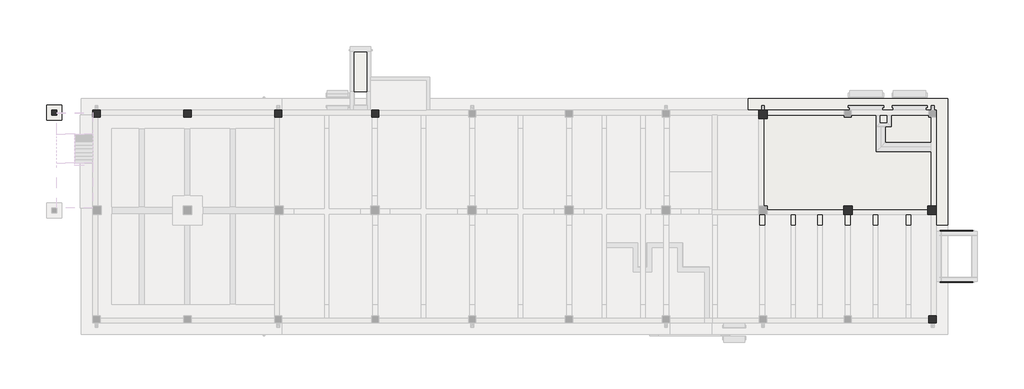
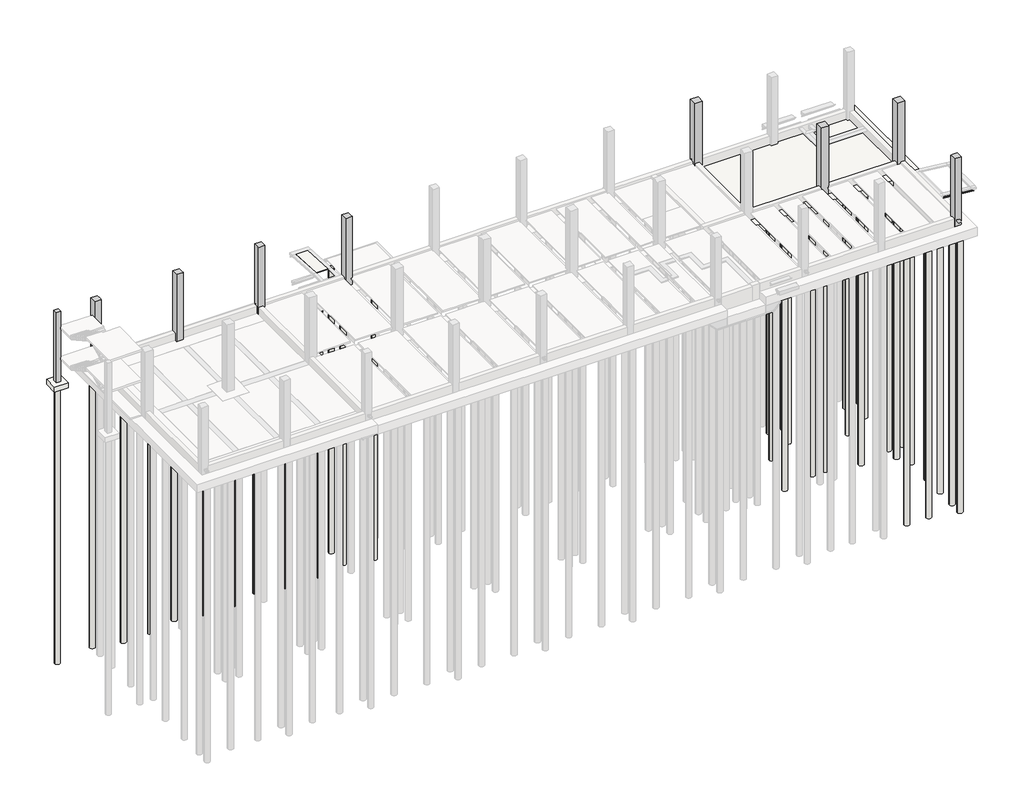
# One storey, part 6 of 7: 46 slabs, 9 columns.
"""IFC4 building model written with IfcOpenShell, lengths in millimetres."""

from ifc_helpers import new_model, si_unit, point, frame, frame_2d, origin, place, context, project, spatial, polyline, circle_curve, trimmed, segment, composite_curve, outline, extrude, faceted_brep, element, save

model = new_model("IFC4")

# Units and contexts
model_context = context("Model", 3, world=origin())
ifc_project = project(units=[si_unit("LENGTHUNIT", "METRE", prefix="MILLI")], contexts=[model_context])

# Site, building, storey
site = spatial("IfcSite", under=ifc_project)
building = spatial("IfcBuilding", under=site)
storey = spatial("IfcBuildingStorey", under=building, Name="H.P.P", Elevation=4500.0)

# Columns
placement = place(None, origin())
element("IfcColumn", 1, ObjectType="RC_Column_Rectangular : H_SC_AR S15_RC Col-AG_700x700_C1", at=placement, inside=storey, context=model_context, shape_type="Brep", body=[
    faceted_brep([(62350.0, -7650.0, 4000.0), (62350.0, -7950.0, 4000.0), (62350.0, -8350.0, 4000.0), (61650.0, -8350.0, 4000.0), (61650.0, -7950.0, 4000.0), (61650.0, -7650.0, 4000.0), (62350.0, -7650.0, 10600.0), (62350.0, -8350.0, 10600.0), (62350.0, -8350.0, 10450.0), (62350.0, -8350.0, 4800.0), (62350.0, -8350.0, 4650.0), (62250.0, -8350.0, 10600.0), (61750.0, -8350.0, 10600.0), (61650.0, -8350.0, 10600.0), (61650.0, -8350.0, 10450.0), (61650.0, -8350.0, 4800.0), (61650.0, -8350.0, 4650.0), (61650.0, -7650.0, 10600.0)], [[[0, 1, 2, 3, 4, 5]], [[2, 1, 0, 6, 7, 8, 9, 10]], [[3, 2, 10, 9, 8, 7, 11, 12, 13, 14, 15, 16]], [[5, 4, 3, 16, 15, 14, 13, 17]], [[0, 5, 17, 6]], [[7, 6, 17, 13, 12, 11]]]),
])
element("IfcColumn", 2, ObjectType="RC_Column_Rectangular : H_SC_AR S15_RC Col-AG_700x700_C1", at=placement, inside=storey, context=model_context, shape_type="Brep", body=[
    faceted_brep([(69300.0, -7650.0, 4000.0), (69300.0, -8350.0, 4000.0), (68900.0, -8350.0, 4000.0), (68600.0, -8350.0, 4000.0), (68600.0, -7950.0, 4000.0), (68600.0, -7650.0, 4000.0), (68900.0, -7650.0, 4000.0), (69300.0, -7650.0, 4800.0), (69300.0, -7650.0, 9900.0), (69300.0, -7650.0, 10600.0), (69300.0, -8350.0, 10600.0), (69300.0, -8350.0, 9900.0), (69300.0, -8350.0, 4800.0), (68900.0, -8350.0, 10600.0), (68600.0, -8350.0, 10600.0), (68600.0, -8350.0, 10450.0), (68600.0, -8350.0, 9800.0), (68600.0, -8350.0, 4800.0), (68600.0, -8350.0, 4650.0), (68600.0, -7650.0, 10600.0)], [[[0, 1, 2, 3, 4, 5, 6]], [[1, 0, 7, 8, 9, 10, 11, 12]], [[3, 2, 1, 12, 11, 10, 13, 14, 15, 16, 17, 18]], [[5, 4, 3, 18, 17, 16, 15, 14, 19]], [[0, 6, 5, 19, 9, 8, 7]], [[10, 9, 19, 14, 13]]]),
])
element("IfcColumn", 3, ObjectType="RC_Column_Rectangular : H_SC_AR S15_RC Col-AG_700x700_C1", at=placement, inside=storey, context=model_context, shape_type="Brep", body=[
    faceted_brep([(55350.0, 300.0, 4000.0), (55350.0, -100.0, 4000.0), (55350.0, -400.0, 4000.0), (55050.0, -400.0, 4000.0), (54650.0, -400.0, 4000.0), (54650.0, -100.0, 4000.0), (54650.0, 300.0, 4000.0), (55350.0, 300.0, 10600.0), (55350.0, -400.0, 10600.0), (55350.0, 300.0, 4800.0), (55350.0, 300.0, 8300.0), (55350.0, 300.0, 9100.0), (54650.0, -400.0, 10600.0), (54650.0, -400.0, 9800.0), (54650.0, -400.0, 4800.0), (54650.0, 300.0, 10600.0), (54650.0, 300.0, 9800.0), (54650.0, 300.0, 4800.0)], [[[0, 1, 2, 3, 4, 5, 6]], [[7, 8, 2, 1, 0, 9, 10, 11]], [[8, 12, 13, 14, 4, 3, 2]], [[12, 15, 16, 17, 6, 5, 4, 14, 13]], [[15, 7, 11, 10, 9, 0, 6, 17, 16]], [[7, 15, 12, 8]]]),
])
element("IfcColumn", 4, ObjectType="RC_Column_Rectangular : H_SC_AR S15_RC Col-AG_600x600_C2", at=placement, inside=storey, context=model_context, shape_type="Brep", body=[
    faceted_brep([(300.0, 300.0, 4100.0), (300.0, -100.0, 4100.0), (300.0, -300.0, 4100.0), (100.0, -300.0, 4100.0), (-300.0, -300.0, 4100.0), (-300.0, -100.0, 4100.0), (-300.0, 300.0, 4100.0), (300.0, 300.0, 4800.0), (300.0, 300.0, 9800.0), (300.0, 300.0, 10600.0), (300.0, -100.0, 10600.0), (300.0, -300.0, 10600.0), (300.0, -300.0, 10450.0), (100.0, -300.0, 10600.0), (-300.0, -300.0, 10600.0), (-300.0, -300.0, 9900.0), (-300.0, -300.0, 4800.0), (-300.0, 300.0, 10600.0), (-300.0, 300.0, 10550.0), (-300.0, 300.0, 9950.0), (-300.0, 300.0, 4630.0)], [[[0, 1, 2, 3, 4, 5, 6]], [[2, 1, 0, 7, 8, 9, 10, 11, 12]], [[4, 3, 2, 12, 11, 13, 14, 15, 16]], [[6, 5, 4, 16, 15, 14, 17, 18, 19, 20]], [[0, 6, 20, 19, 18, 17, 9, 8, 7]], [[17, 14, 13, 11, 10, 9]]]),
])
element("IfcColumn", 5, ObjectType="RC_Column_Rectangular : H_SC_AR S15_RC Col-AG_600x600_C2", at=placement, inside=storey, context=model_context, shape_type="Brep", body=[
    faceted_brep([(7800.0, 300.0, 4100.0), (7800.0, -100.0, 4100.0), (7800.0, -300.0, 4100.0), (7200.0, -300.0, 4100.0), (7200.0, -100.0, 4100.0), (7200.0, 300.0, 4100.0), (7800.0, 300.0, 4800.0), (7800.0, 300.0, 9800.0), (7800.0, 300.0, 10600.0), (7800.0, -100.0, 10600.0), (7800.0, -300.0, 10600.0), (7800.0, -300.0, 10450.0), (7750.0, -300.0, 10600.0), (7250.0, -300.0, 10600.0), (7200.0, -300.0, 10600.0), (7200.0, -300.0, 10450.0), (7200.0, -100.0, 10600.0), (7200.0, 300.0, 10600.0), (7200.0, 300.0, 9800.0), (7200.0, 300.0, 4800.0)], [[[0, 1, 2, 3, 4, 5]], [[2, 1, 0, 6, 7, 8, 9, 10, 11]], [[3, 2, 11, 10, 12, 13, 14, 15]], [[5, 4, 3, 15, 14, 16, 17, 18, 19]], [[0, 5, 19, 18, 17, 8, 7, 6]], [[8, 17, 16, 14, 13, 12, 10, 9]]]),
])
element("IfcColumn", 6, ObjectType="RC_Column_Rectangular : H_SC_AR S15_RC Col-AG_600x600_C2", at=placement, inside=storey, context=model_context, shape_type="Brep", body=[
    faceted_brep([(15300.0, 300.0, 4100.0), (15300.0, -300.0, 4100.0), (15100.0, -300.0, 4100.0), (14700.0, -300.0, 4100.0), (14700.0, -100.0, 4100.0), (14700.0, 300.0, 4100.0), (15300.0, 300.0, 4800.0), (15300.0, 300.0, 9800.0), (15300.0, 300.0, 10600.0), (15300.0, -100.0, 10600.0), (15300.0, -300.0, 10600.0), (15300.0, -300.0, 10450.0), (15300.0, -300.0, 4800.0), (15300.0, -300.0, 4650.0), (15200.0, -300.0, 10600.0), (14700.0, -300.0, 10600.0), (14700.0, -300.0, 10450.0), (14700.0, -300.0, 4800.0), (14700.0, -100.0, 10600.0), (14700.0, 300.0, 10600.0), (14700.0, 300.0, 9800.0), (14700.0, 300.0, 4800.0)], [[[0, 1, 2, 3, 4, 5]], [[1, 0, 6, 7, 8, 9, 10, 11, 12, 13]], [[3, 2, 1, 13, 12, 11, 10, 14, 15, 16, 17]], [[5, 4, 3, 17, 16, 15, 18, 19, 20, 21]], [[0, 5, 21, 20, 19, 8, 7, 6]], [[8, 19, 18, 15, 14, 10, 9]]]),
])
element("IfcColumn", 7, ObjectType="RC_Column_Rectangular : H_SC_AR S15_RC Col-AG_600x600_C2", at=placement, inside=storey, context=model_context, shape_type="Brep", body=[
    faceted_brep([(23300.0, 300.0, 4000.0), (23300.0, -100.0, 4000.0), (23300.0, -300.0, 4000.0), (22700.0, -300.0, 4000.0), (22700.0, -100.0, 4000.0), (22700.0, 300.0, 4000.0), (23300.0, 300.0, 4800.0), (23300.0, 300.0, 9800.0), (23300.0, 300.0, 10600.0), (23300.0, -100.0, 10600.0), (23300.0, -300.0, 10600.0), (23300.0, -300.0, 10450.0), (23300.0, -300.0, 4800.0), (23300.0, -300.0, 4650.0), (23200.0, -300.0, 10600.0), (22700.0, -300.0, 10600.0), (22700.0, -300.0, 10450.0), (22700.0, -300.0, 4800.0), (22700.0, -300.0, 4650.0), (22700.0, -100.0, 10600.0), (22700.0, 300.0, 10600.0), (22700.0, 300.0, 4800.0)], [[[0, 1, 2, 3, 4, 5]], [[2, 1, 0, 6, 7, 8, 9, 10, 11, 12, 13]], [[3, 2, 13, 12, 11, 10, 14, 15, 16, 17, 18]], [[5, 4, 3, 18, 17, 16, 15, 19, 20, 21]], [[0, 5, 21, 20, 8, 7, 6]], [[8, 20, 19, 15, 14, 10, 9]]]),
])
element("IfcColumn", 8, ObjectType="RC_Column_Rectangular : H_SC_AR S15_RC Col-AG_600x600_C2", at=placement, inside=storey, context=model_context, shape_type="Brep", body=[
    faceted_brep([(69300.0, -16700.0, 4000.0), (69300.0, -17300.0, 4000.0), (68700.0, -17300.0, 4000.0), (68700.0, -16900.0, 4000.0), (68700.0, -16700.0, 4000.0), (68900.0, -16700.0, 4000.0), (69300.0, -16700.0, 4800.0), (69300.0, -16700.0, 9900.0), (69300.0, -16700.0, 10600.0), (69300.0, -17300.0, 10600.0), (68700.0, -17300.0, 10600.0), (68700.0, -17300.0, 9800.0), (68700.0, -17300.0, 4800.0), (68700.0, -16900.0, 10600.0), (68700.0, -16700.0, 10600.0), (68700.0, -16700.0, 10450.0), (68700.0, -16700.0, 4800.0), (68700.0, -16700.0, 4650.0), (68900.0, -16700.0, 10600.0)], [[[0, 1, 2, 3, 4, 5]], [[1, 0, 6, 7, 8, 9]], [[2, 1, 9, 10, 11, 12]], [[4, 3, 2, 12, 11, 10, 13, 14, 15, 16, 17]], [[0, 5, 4, 17, 16, 15, 14, 18, 8, 7, 6]], [[9, 8, 18, 14, 13, 10]]]),
])
element("IfcColumn", 9, ObjectType="RC_Column_Rectangular : H_SC_AR S15_RC Col-AG_400x400_C3", at=placement, inside=storey, context=model_context, shape_type="Brep", body=[
    faceted_brep([(-3300.0, 300.0, 3800.0), (-3300.0, -100.0, 3800.0), (-3700.0, -100.0, 3800.0), (-3700.0, 300.0, 3800.0), (-3300.0, 300.0, 10600.0), (-3300.0, -100.0, 10600.0), (-3300.0, -100.0, 10550.0), (-3300.0, -100.0, 9950.0), (-3300.0, -100.0, 7590.0), (-3300.0, -100.0, 6990.0), (-3300.0, -100.0, 4630.0), (-3300.0, -100.0, 4100.0), (-3300.0, -100.0, 4030.0), (-3300.0, 300.0, 4100.0), (-3300.0, 300.0, 4630.0), (-3300.0, 300.0, 9950.0), (-3300.0, 300.0, 10550.0), (-3700.0, -100.0, 10600.0), (-3700.0, -100.0, 10550.0), (-3700.0, -100.0, 9950.0), (-3700.0, -100.0, 7590.0), (-3700.0, -100.0, 6990.0), (-3700.0, -100.0, 4630.0), (-3700.0, -100.0, 4030.0), (-3700.0, 300.0, 10600.0)], [[[0, 1, 2, 3]], [[4, 5, 6, 7, 8, 9, 10, 11, 12, 1, 0, 13, 14, 15, 16]], [[5, 17, 18, 19, 20, 21, 22, 23, 2, 1, 12, 11, 10, 9, 8, 7, 6]], [[17, 24, 3, 2, 23, 22, 21, 20, 19, 18]], [[24, 4, 16, 15, 14, 13, 0, 3]], [[4, 24, 17, 5]]]),
])

# Slabs
element("IfcSlab", 10, ObjectType="H_SF_AR S18_MAT_T800_MF1", at=placement, inside=storey, context=model_context, shape_type="Brep", body=[
    faceted_brep([(70250.0, 1249.9999999, 3200.0), (70250.0, -9250.0000001, 3200.0), (67750.0000002, -9250.0000001, 3200.0), (53749.9998007, -9250.0000001, 3200.0), (53749.9998007, -6750.0000001, 3200.0), (53749.9998007, -1250.0000001, 3200.0), (53749.9998007, 1249.9999999, 3200.0), (70250.0, -9250.0000001, 4000.0), (70250.0, 1249.9999999, 4000.0), (53749.9998007, 1249.9999999, 4000.0), (53749.9998007, -1250.0000001, 4000.0), (53749.9998007, -6750.0000001, 4000.0), (53749.9998007, -9250.0000001, 4000.0), (67750.0000002, -9250.0000001, 4000.0)], [[[0, 1, 2, 3, 4, 5, 6]], [[7, 8, 9, 10, 11, 12, 13]], [[1, 0, 8, 7]], [[1, 7, 13, 12, 3, 2]], [[3, 12, 11, 10, 9, 6, 5, 4]], [[0, 6, 9, 8]]]),
])
element("IfcSlab", 11, ObjectType="H_SF_AR_S18_Lean_T50", at=placement, inside=storey, context=model_context, shape_type="Brep", body=[
    faceted_brep([(72401.1499651, -13950.0, 4178.1393567), (69580.8773013, -13950.0, 4460.1666231), (69580.8773013, -13700.0, 4460.1666231), (72401.1499651, -13700.0, 4178.1393567), (69626.5585541, -13700.0, 4505.847876), (69626.5585541, -13850.0, 4505.847876), (69626.5585541, -13950.0, 4505.847876), (72345.3173228, -13950.0, 4233.9719991), (72345.3173228, -13850.0, 4233.9719991), (72345.3173228, -13700.0, 4233.9719991)], [[[0, 1, 2, 3]], [[4, 5, 6, 7, 8, 9]], [[1, 0, 7, 6]], [[3, 2, 4, 9]], [[5, 4, 2, 1, 6]], [[0, 3, 9, 8, 7]]]),
])
element("IfcSlab", 12, ObjectType="H_SF_AR_S18_Lean_T50", at=placement, inside=storey, context=model_context, shape_type="Brep", body=[
    faceted_brep([(69580.8773013, -9650.0, 4460.1666231), (72401.1499651, -9650.0, 4178.1393567), (72401.1499651, -9900.0, 4178.1393567), (69580.8773013, -9900.0, 4460.1666231), (72345.3173228, -9750.0, 4233.9719991), (72345.3173228, -9650.0, 4233.9719991), (69626.5585541, -9650.0, 4505.847876), (69626.5585541, -9750.0, 4505.847876), (69626.5585541, -9900.0, 4505.847876), (72345.3173228, -9900.0, 4233.9719991)], [[[0, 1, 2, 3]], [[4, 5, 6, 7, 8, 9]], [[1, 0, 6, 5]], [[3, 2, 9, 8]], [[2, 1, 5, 4, 9]], [[0, 3, 8, 7, 6]]]),
])
element("IfcSlab", 13, ObjectType="H_SF_AR_S18_Lean_T50", at=placement, inside=storey, context=model_context, shape_type="Brep", body=[
    faceted_brep([(22338.0, 5100.0, 4329.5560483), (22338.0, 1800.0, 4549.5560483), (21238.0, 1800.0, 4549.5560483), (21238.0, 5100.0, 4329.5560483), (22338.0, 5100.0, 4379.6670362), (21238.0, 5100.0, 4379.6670362), (21238.0, 1800.0, 4599.6670362), (22338.0, 1800.0, 4599.6670362), (22338.0, 1800.0, 4550.0), (21238.0, 1800.0, 4550.0)], [[[0, 1, 2, 3]], [[4, 5, 6, 7]], [[1, 0, 4, 7, 8]], [[2, 1, 8, 7, 6, 9]], [[3, 2, 9, 6, 5]], [[0, 3, 5, 4]]]),
])
element("IfcSlab", 14, ObjectType="Foundation Rectangular (Non-Pile) : H_SF_AR S18_Ret Fdn_1250x1250xT500_F2", at=placement, inside=storey, context=model_context, shape_type="SweptSolid", body=[
    extrude(outline(polyline([(-2875.0, 725.0), (-2875.0, -525.0), (-4125.0, -525.0), (-4125.0, 725.0), (-2875.0, 725.0)])), frame((0.0, 0.0, 3300.0), z_axis=(0.0, 0.0, 1.0), x_axis=(1.0, 0.0, 0.0)), (0.0, 0.0, 1.0), 500.0),
])
element("IfcSlab", 15, ObjectType="PILE : H_FL_AR S19_Pile_D500_L26.9", at=placement, inside=storey, context=model_context, shape_type="SweptSolid", body=[
    extrude(outline(composite_curve([segment(trimmed(circle_curve(frame_2d((-3500.0, 100.0)), 250.0), [point((-3250.0, 100.0))], [point((-3750.0, 100.0))], False, "CARTESIAN"), True, "CONTINUOUS"), segment(trimmed(circle_curve(frame_2d((-3500.0, 100.0)), 250.0), [point((-3750.0, 100.0))], [point((-3250.0, 100.0))], False, "CARTESIAN"), True, "CONTINUOUS")], self_intersect=False)), frame((0.0, 0.0, 3300.0), z_axis=(0.0, 0.0, 1.0), x_axis=(1.0, 0.0, 0.0)), (0.0, 0.0, 1.0), 100.0),
    extrude(outline(composite_curve([segment(trimmed(circle_curve(frame_2d((-3500.0, 100.0)), 250.0), [point((-3750.0, 100.0))], [point((-3250.0, 100.0))], False, "CARTESIAN"), True, "CONTINUOUS"), segment(trimmed(circle_curve(frame_2d((-3500.0, 100.0)), 250.0), [point((-3250.0, 100.0))], [point((-3750.0, 100.0))], False, "CARTESIAN"), True, "CONTINUOUS")], self_intersect=False)), frame((0.0, 0.0, -23500.0), z_axis=(0.0, 0.0, 1.0), x_axis=(1.0, 0.0, 0.0)), (0.0, 0.0, 1.0), 26750.0),
])
element("IfcSlab", 16, ObjectType="PILE : H_FL_AR S19_Pile_D500_L26.9", at=placement, inside=storey, context=model_context, shape_type="SweptSolid", body=[
    extrude(outline(composite_curve([segment(trimmed(circle_curve(frame_2d((0.0, 624.9999997)), 250.0), [point((-250.0, 624.9999997))], [point((250.0, 624.9999997))], False, "CARTESIAN"), True, "CONTINUOUS"), segment(trimmed(circle_curve(frame_2d((0.0, 624.9999997)), 250.0), [point((250.0, 624.9999997))], [point((-250.0, 624.9999997))], False, "CARTESIAN"), True, "CONTINUOUS")], self_intersect=False)), frame((0.0, 0.0, -23500.0), z_axis=(0.0, 0.0, 1.0), x_axis=(1.0, 0.0, 0.0)), (0.0, 0.0, 1.0), 26750.0),
])
element("IfcSlab", 17, ObjectType="PILE : H_FL_AR S19_Pile_D500_L26.9", at=placement, inside=storey, context=model_context, shape_type="SweptSolid", body=[
    extrude(outline(composite_curve([segment(trimmed(circle_curve(frame_2d((2500.0000001, 0.0)), 250.0), [point((2250.0000001, 0.0))], [point((2750.0000001, 0.0))], False, "CARTESIAN"), True, "CONTINUOUS"), segment(trimmed(circle_curve(frame_2d((2500.0000001, 0.0)), 250.0), [point((2750.0000001, 0.0))], [point((2250.0000001, 0.0))], False, "CARTESIAN"), True, "CONTINUOUS")], self_intersect=False)), frame((0.0, 0.0, -23500.0), z_axis=(0.0, 0.0, 1.0), x_axis=(1.0, 0.0, 0.0)), (0.0, 0.0, 1.0), 26750.0),
])
element("IfcSlab", 18, ObjectType="PILE : H_FL_AR S19_Pile_D500_L26.9", at=placement, inside=storey, context=model_context, shape_type="SweptSolid", body=[
    extrude(outline(composite_curve([segment(trimmed(circle_curve(frame_2d((5000.0000002, 0.0)), 250.0), [point((4750.0000002, 0.0))], [point((5250.0000002, 0.0))], False, "CARTESIAN"), True, "CONTINUOUS"), segment(trimmed(circle_curve(frame_2d((5000.0000002, 0.0)), 250.0), [point((5250.0000002, 0.0))], [point((4750.0000002, 0.0))], False, "CARTESIAN"), True, "CONTINUOUS")], self_intersect=False)), frame((0.0, 0.0, -23500.0), z_axis=(0.0, 0.0, 1.0), x_axis=(1.0, 0.0, 0.0)), (0.0, 0.0, 1.0), 26750.0),
])
element("IfcSlab", 19, ObjectType="PILE : H_FL_AR S19_Pile_D500_L26.9", at=placement, inside=storey, context=model_context, shape_type="SweptSolid", body=[
    extrude(outline(composite_curve([segment(trimmed(circle_curve(frame_2d((7500.0, 625.0)), 250.0), [point((7250.0, 625.0))], [point((7750.0, 625.0))], False, "CARTESIAN"), True, "CONTINUOUS"), segment(trimmed(circle_curve(frame_2d((7500.0, 625.0)), 250.0), [point((7750.0, 625.0))], [point((7250.0, 625.0))], False, "CARTESIAN"), True, "CONTINUOUS")], self_intersect=False)), frame((0.0, 0.0, -23500.0), z_axis=(0.0, 0.0, 1.0), x_axis=(1.0, 0.0, 0.0)), (0.0, 0.0, 1.0), 26750.0),
])
element("IfcSlab", 20, ObjectType="PILE : H_FL_AR S19_Pile_D500_L26.9", at=placement, inside=storey, context=model_context, shape_type="SweptSolid", body=[
    extrude(outline(composite_curve([segment(trimmed(circle_curve(frame_2d((10000.0000005, 0.0)), 250.0), [point((9750.0000005, 0.0))], [point((10250.0000005, 0.0))], False, "CARTESIAN"), True, "CONTINUOUS"), segment(trimmed(circle_curve(frame_2d((10000.0000005, 0.0)), 250.0), [point((10250.0000005, 0.0))], [point((9750.0000005, 0.0))], False, "CARTESIAN"), True, "CONTINUOUS")], self_intersect=False)), frame((0.0, 0.0, -23500.0), z_axis=(0.0, 0.0, 1.0), x_axis=(1.0, 0.0, 0.0)), (0.0, 0.0, 1.0), 26750.0),
])
element("IfcSlab", 21, ObjectType="PILE : H_FL_AR S19_Pile_D500_L26.9", at=placement, inside=storey, context=model_context, shape_type="SweptSolid", body=[
    extrude(outline(composite_curve([segment(trimmed(circle_curve(frame_2d((12500.0000007, 0.0)), 250.0), [point((12250.0000007, 0.0))], [point((12750.0000007, 0.0))], False, "CARTESIAN"), True, "CONTINUOUS"), segment(trimmed(circle_curve(frame_2d((12500.0000007, 0.0)), 250.0), [point((12750.0000007, 0.0))], [point((12250.0000007, 0.0))], False, "CARTESIAN"), True, "CONTINUOUS")], self_intersect=False)), frame((0.0, 0.0, -23500.0), z_axis=(0.0, 0.0, 1.0), x_axis=(1.0, 0.0, 0.0)), (0.0, 0.0, 1.0), 26750.0),
])
element("IfcSlab", 22, ObjectType="PILE : H_FL_AR S19_Pile_D500_L26.8", at=placement, inside=storey, context=model_context, shape_type="SweptSolid", body=[
    extrude(outline(composite_curve([segment(trimmed(circle_curve(frame_2d((14999.9999999, 625.0000001)), 250.0), [point((15249.9999999, 625.0000001))], [point((14749.9999999, 625.0000001))], False, "CARTESIAN"), True, "CONTINUOUS"), segment(trimmed(circle_curve(frame_2d((14999.9999999, 625.0000001)), 250.0), [point((14749.9999999, 625.0000001))], [point((15249.9999999, 625.0000001))], False, "CARTESIAN"), True, "CONTINUOUS")], self_intersect=False)), frame((0.0, 0.0, 3200.0), z_axis=(0.0, 0.0, 1.0), x_axis=(1.0, 0.0, 0.0)), (0.0, 0.0, 1.0), 100.0),
    extrude(outline(composite_curve([segment(trimmed(circle_curve(frame_2d((14999.9999999, 625.0000001)), 250.0), [point((14749.9999999, 625.0000001))], [point((15249.9999999, 625.0000001))], False, "CARTESIAN"), True, "CONTINUOUS"), segment(trimmed(circle_curve(frame_2d((14999.9999999, 625.0000001)), 250.0), [point((15249.9999999, 625.0000001))], [point((14749.9999999, 625.0000001))], False, "CARTESIAN"), True, "CONTINUOUS")], self_intersect=False)), frame((0.0, 0.0, -23500.0), z_axis=(0.0, 0.0, 1.0), x_axis=(1.0, 0.0, 0.0)), (0.0, 0.0, 1.0), 26650.0),
])
element("IfcSlab", 23, ObjectType="PILE : H_FL_AR S19_Pile_D500_L26.8", at=placement, inside=storey, context=model_context, shape_type="SweptSolid", body=[
    extrude(outline(composite_curve([segment(trimmed(circle_curve(frame_2d((17500.0000007, 0.0)), 250.0), [point((17250.0000007, 0.0))], [point((17750.0000007, 0.0))], False, "CARTESIAN"), True, "CONTINUOUS"), segment(trimmed(circle_curve(frame_2d((17500.0000007, 0.0)), 250.0), [point((17750.0000007, 0.0))], [point((17250.0000007, 0.0))], False, "CARTESIAN"), True, "CONTINUOUS")], self_intersect=False)), frame((0.0, 0.0, -23500.0), z_axis=(0.0, 0.0, 1.0), x_axis=(1.0, 0.0, 0.0)), (0.0, 0.0, 1.0), 26650.0),
])
element("IfcSlab", 24, ObjectType="PILE : H_FL_AR S19_Pile_D500_L26.8", at=placement, inside=storey, context=model_context, shape_type="SweptSolid", body=[
    extrude(outline(composite_curve([segment(trimmed(circle_curve(frame_2d((20499.9999999, 0.0)), 250.0), [point((20249.9999999, 0.0))], [point((20749.9999999, 0.0))], False, "CARTESIAN"), True, "CONTINUOUS"), segment(trimmed(circle_curve(frame_2d((20499.9999999, 0.0)), 250.0), [point((20749.9999999, 0.0))], [point((20249.9999999, 0.0))], False, "CARTESIAN"), True, "CONTINUOUS")], self_intersect=False)), frame((0.0, 0.0, -23500.0), z_axis=(0.0, 0.0, 1.0), x_axis=(1.0, 0.0, 0.0)), (0.0, 0.0, 1.0), 26650.0),
])
element("IfcSlab", 25, ObjectType="PILE : H_FL_AR S19_Pile_D500_L26.8", at=placement, inside=storey, context=model_context, shape_type="SweptSolid", body=[
    extrude(outline(composite_curve([segment(trimmed(circle_curve(frame_2d((23000.0, 624.9999997)), 250.0), [point((22750.0, 624.9999997))], [point((23250.0, 624.9999997))], False, "CARTESIAN"), True, "CONTINUOUS"), segment(trimmed(circle_curve(frame_2d((23000.0, 624.9999997)), 250.0), [point((23250.0, 624.9999997))], [point((22750.0, 624.9999997))], False, "CARTESIAN"), True, "CONTINUOUS")], self_intersect=False)), frame((0.0, 0.0, -23500.0), z_axis=(0.0, 0.0, 1.0), x_axis=(1.0, 0.0, 0.0)), (0.0, 0.0, 1.0), 26650.0),
])
element("IfcSlab", 26, ObjectType="PILE : H_FL_AR S19_Pile_D500_L27.7", at=placement, inside=storey, context=model_context, shape_type="SweptSolid", body=[
    extrude(outline(composite_curve([segment(trimmed(circle_curve(frame_2d((23000.0, 2500.0)), 250.0), [point((22750.0, 2500.0))], [point((23250.0, 2500.0))], False, "CARTESIAN"), True, "CONTINUOUS"), segment(trimmed(circle_curve(frame_2d((23000.0, 2500.0)), 250.0), [point((23250.0, 2500.0))], [point((22750.0, 2500.0))], False, "CARTESIAN"), True, "CONTINUOUS")], self_intersect=False)), frame((0.0, 0.0, -23500.0), z_axis=(0.0, 0.0, 1.0), x_axis=(1.0, 0.0, 0.0)), (0.0, 0.0, 1.0), 27550.0),
])
element("IfcSlab", 27, ObjectType="PILE : H_FL_AR S19_Pile_D500_L26.8", at=placement, inside=storey, context=model_context, shape_type="SweptSolid", body=[
    extrude(outline(composite_curve([segment(trimmed(circle_curve(frame_2d((25500.0000013, 0.0)), 250.0), [point((25250.0000013, 0.0))], [point((25750.0000013, 0.0))], False, "CARTESIAN"), True, "CONTINUOUS"), segment(trimmed(circle_curve(frame_2d((25500.0000013, 0.0)), 250.0), [point((25750.0000013, 0.0))], [point((25250.0000013, 0.0))], False, "CARTESIAN"), True, "CONTINUOUS")], self_intersect=False)), frame((0.0, 0.0, -23500.0), z_axis=(0.0, 0.0, 1.0), x_axis=(1.0, 0.0, 0.0)), (0.0, 0.0, 1.0), 26650.0),
])
element("IfcSlab", 28, ObjectType="PILE : H_FL_AR S19_Pile_D500_L26.8", at=placement, inside=storey, context=model_context, shape_type="SweptSolid", body=[
    extrude(outline(composite_curve([segment(trimmed(circle_curve(frame_2d((64499.9999998, -17000.0)), 250.0), [point((64249.9999998, -17000.0))], [point((64749.9999998, -17000.0))], False, "CARTESIAN"), True, "CONTINUOUS"), segment(trimmed(circle_curve(frame_2d((64499.9999998, -17000.0)), 250.0), [point((64749.9999998, -17000.0))], [point((64249.9999998, -17000.0))], False, "CARTESIAN"), True, "CONTINUOUS")], self_intersect=False)), frame((0.0, 0.0, -23500.0), z_axis=(0.0, 0.0, 1.0), x_axis=(1.0, 0.0, 0.0)), (0.0, 0.0, 1.0), 26650.0),
])
element("IfcSlab", 29, ObjectType="PILE : H_FL_AR S19_Pile_D500_L26.8", at=placement, inside=storey, context=model_context, shape_type="SweptSolid", body=[
    extrude(outline(composite_curve([segment(trimmed(circle_curve(frame_2d((66500.0, -17000.0)), 250.0), [point((66250.0, -17000.0))], [point((66750.0, -17000.0))], False, "CARTESIAN"), True, "CONTINUOUS"), segment(trimmed(circle_curve(frame_2d((66500.0, -17000.0)), 250.0), [point((66750.0, -17000.0))], [point((66250.0, -17000.0))], False, "CARTESIAN"), True, "CONTINUOUS")], self_intersect=False)), frame((0.0, 0.0, -23500.0), z_axis=(0.0, 0.0, 1.0), x_axis=(1.0, 0.0, 0.0)), (0.0, 0.0, 1.0), 26650.0),
])
element("IfcSlab", 30, ObjectType="PILE : H_FL_AR S19_Pile_D500_L26.8", at=placement, inside=storey, context=model_context, shape_type="SweptSolid", body=[
    extrude(outline(composite_curve([segment(trimmed(circle_curve(frame_2d((69000.0, -17625.0000002)), 250.0), [point((68750.0, -17625.0000002))], [point((69250.0, -17625.0000002))], False, "CARTESIAN"), True, "CONTINUOUS"), segment(trimmed(circle_curve(frame_2d((69000.0, -17625.0000002)), 250.0), [point((69250.0, -17625.0000002))], [point((68750.0, -17625.0000002))], False, "CARTESIAN"), True, "CONTINUOUS")], self_intersect=False)), frame((0.0, 0.0, -23500.0), z_axis=(0.0, 0.0, 1.0), x_axis=(1.0, 0.0, 0.0)), (0.0, 0.0, 1.0), 26650.0),
])
element("IfcSlab", 31, ObjectType="PILE : H_FL_AR S19_Pile_D500_L26.8", at=placement, inside=storey, context=model_context, shape_type="SweptSolid", body=[
    extrude(outline(composite_curve([segment(trimmed(circle_curve(frame_2d((69000.0, -16375.0000006)), 250.0), [point((68750.0, -16375.0000006))], [point((69250.0, -16375.0000006))], False, "CARTESIAN"), True, "CONTINUOUS"), segment(trimmed(circle_curve(frame_2d((69000.0, -16375.0000006)), 250.0), [point((69250.0, -16375.0000006))], [point((68750.0, -16375.0000006))], False, "CARTESIAN"), True, "CONTINUOUS")], self_intersect=False)), frame((0.0, 0.0, -23500.0), z_axis=(0.0, 0.0, 1.0), x_axis=(1.0, 0.0, 0.0)), (0.0, 0.0, 1.0), 26650.0),
])
element("IfcSlab", 32, ObjectType="PILE : H_FL_AR S19_Pile_D500_L26.8", at=placement, inside=storey, context=model_context, shape_type="SweptSolid", body=[
    extrude(outline(composite_curve([segment(trimmed(circle_curve(frame_2d((69000.0, -14499.9999999)), 250.0), [point((68750.0, -14499.9999999))], [point((69250.0, -14499.9999999))], False, "CARTESIAN"), True, "CONTINUOUS"), segment(trimmed(circle_curve(frame_2d((69000.0, -14499.9999999)), 250.0), [point((69250.0, -14499.9999999))], [point((68750.0, -14499.9999999))], False, "CARTESIAN"), True, "CONTINUOUS")], self_intersect=False)), frame((0.0, 0.0, -23500.0), z_axis=(0.0, 0.0, 1.0), x_axis=(1.0, 0.0, 0.0)), (0.0, 0.0, 1.0), 26650.0),
])
element("IfcSlab", 33, ObjectType="PILE : H_FL_AR S19_Pile_D500_L26.8", at=placement, inside=storey, context=model_context, shape_type="SweptSolid", body=[
    extrude(outline(composite_curve([segment(trimmed(circle_curve(frame_2d((69000.0, -12375.0000001)), 250.0), [point((68750.0, -12375.0000001))], [point((69250.0, -12375.0000001))], False, "CARTESIAN"), True, "CONTINUOUS"), segment(trimmed(circle_curve(frame_2d((69000.0, -12375.0000001)), 250.0), [point((69250.0, -12375.0000001))], [point((68750.0, -12375.0000001))], False, "CARTESIAN"), True, "CONTINUOUS")], self_intersect=False)), frame((0.0, 0.0, -23500.0), z_axis=(0.0, 0.0, 1.0), x_axis=(1.0, 0.0, 0.0)), (0.0, 0.0, 1.0), 26650.0),
])
element("IfcSlab", 34, ObjectType="PILE : H_FL_AR S19_Pile_D500_L26.8", at=placement, inside=storey, context=model_context, shape_type="SweptSolid", body=[
    extrude(outline(composite_curve([segment(trimmed(circle_curve(frame_2d((69000.0, -9874.9999999)), 250.0), [point((68750.0, -9874.9999999))], [point((69250.0, -9874.9999999))], False, "CARTESIAN"), True, "CONTINUOUS"), segment(trimmed(circle_curve(frame_2d((69000.0, -9874.9999999)), 250.0), [point((69250.0, -9874.9999999))], [point((68750.0, -9874.9999999))], False, "CARTESIAN"), True, "CONTINUOUS")], self_intersect=False)), frame((0.0, 0.0, -23500.0), z_axis=(0.0, 0.0, 1.0), x_axis=(1.0, 0.0, 0.0)), (0.0, 0.0, 1.0), 26650.0),
])
element("IfcSlab", 35, ObjectType="PILE : H_FL_AR S19_Pile_D500_L26.8", at=placement, inside=storey, context=model_context, shape_type="SweptSolid", body=[
    extrude(outline(composite_curve([segment(trimmed(circle_curve(frame_2d((69625.0, -8625.0)), 250.0), [point((69375.0, -8625.0))], [point((69875.0, -8625.0))], False, "CARTESIAN"), True, "CONTINUOUS"), segment(trimmed(circle_curve(frame_2d((69625.0, -8625.0)), 250.0), [point((69875.0, -8625.0))], [point((69375.0, -8625.0))], False, "CARTESIAN"), True, "CONTINUOUS")], self_intersect=False)), frame((0.0, 0.0, -23500.0), z_axis=(0.0, 0.0, 1.0), x_axis=(1.0, 0.0, 0.0)), (0.0, 0.0, 1.0), 26650.0),
])
element("IfcSlab", 36, ObjectType="PILE : H_FL_AR S19_Pile_D500_L26.8", at=placement, inside=storey, context=model_context, shape_type="SweptSolid", body=[
    extrude(outline(composite_curve([segment(trimmed(circle_curve(frame_2d((69625.0, -7375.0)), 250.0), [point((69375.0, -7375.0))], [point((69875.0, -7375.0))], False, "CARTESIAN"), True, "CONTINUOUS"), segment(trimmed(circle_curve(frame_2d((69625.0, -7375.0)), 250.0), [point((69875.0, -7375.0))], [point((69375.0, -7375.0))], False, "CARTESIAN"), True, "CONTINUOUS")], self_intersect=False)), frame((0.0, 0.0, -23500.0), z_axis=(0.0, 0.0, 1.0), x_axis=(1.0, 0.0, 0.0)), (0.0, 0.0, 1.0), 26650.0),
])
element("IfcSlab", 37, ObjectType="PILE : H_FL_AR S19_Pile_D500_L26.8", at=placement, inside=storey, context=model_context, shape_type="SweptSolid", body=[
    extrude(outline(composite_curve([segment(trimmed(circle_curve(frame_2d((68375.0, -7375.0)), 250.0), [point((68125.0, -7375.0))], [point((68625.0, -7375.0))], False, "CARTESIAN"), True, "CONTINUOUS"), segment(trimmed(circle_curve(frame_2d((68375.0, -7375.0)), 250.0), [point((68625.0, -7375.0))], [point((68125.0, -7375.0))], False, "CARTESIAN"), True, "CONTINUOUS")], self_intersect=False)), frame((0.0, 0.0, -23500.0), z_axis=(0.0, 0.0, 1.0), x_axis=(1.0, 0.0, 0.0)), (0.0, 0.0, 1.0), 26650.0),
])
element("IfcSlab", 38, ObjectType="PILE : H_FL_AR S19_Pile_D500_L26.8", at=placement, inside=storey, context=model_context, shape_type="SweptSolid", body=[
    extrude(outline(composite_curve([segment(trimmed(circle_curve(frame_2d((68375.0, -8625.0)), 250.0), [point((68125.0, -8625.0))], [point((68625.0, -8625.0))], False, "CARTESIAN"), True, "CONTINUOUS"), segment(trimmed(circle_curve(frame_2d((68375.0, -8625.0)), 250.0), [point((68625.0, -8625.0))], [point((68125.0, -8625.0))], False, "CARTESIAN"), True, "CONTINUOUS")], self_intersect=False)), frame((0.0, 0.0, -23500.0), z_axis=(0.0, 0.0, 1.0), x_axis=(1.0, 0.0, 0.0)), (0.0, 0.0, 1.0), 26650.0),
])
element("IfcSlab", 39, ObjectType="PILE : H_FL_AR S19_Pile_D500_L26.8", at=placement, inside=storey, context=model_context, shape_type="SweptSolid", body=[
    extrude(outline(composite_curve([segment(trimmed(circle_curve(frame_2d((65500.0, -8000.0)), 250.0), [point((65250.0, -8000.0))], [point((65750.0, -8000.0))], False, "CARTESIAN"), True, "CONTINUOUS"), segment(trimmed(circle_curve(frame_2d((65500.0, -8000.0)), 250.0), [point((65750.0, -8000.0))], [point((65250.0, -8000.0))], False, "CARTESIAN"), True, "CONTINUOUS")], self_intersect=False)), frame((0.0, 0.0, -23500.0), z_axis=(0.0, 0.0, 1.0), x_axis=(1.0, 0.0, 0.0)), (0.0, 0.0, 1.0), 26650.0),
])
element("IfcSlab", 40, ObjectType="PILE : H_FL_AR S19_Pile_D500_L26.8", at=placement, inside=storey, context=model_context, shape_type="SweptSolid", body=[
    extrude(outline(composite_curve([segment(trimmed(circle_curve(frame_2d((62625.0000001, -7375.0)), 250.0), [point((62375.0000001, -7375.0))], [point((62875.0000001, -7375.0))], False, "CARTESIAN"), True, "CONTINUOUS"), segment(trimmed(circle_curve(frame_2d((62625.0000001, -7375.0)), 250.0), [point((62875.0000001, -7375.0))], [point((62375.0000001, -7375.0))], False, "CARTESIAN"), True, "CONTINUOUS")], self_intersect=False)), frame((0.0, 0.0, -23500.0), z_axis=(0.0, 0.0, 1.0), x_axis=(1.0, 0.0, 0.0)), (0.0, 0.0, 1.0), 26650.0),
])
element("IfcSlab", 41, ObjectType="PILE : H_FL_AR S19_Pile_D500_L26.8", at=placement, inside=storey, context=model_context, shape_type="SweptSolid", body=[
    extrude(outline(composite_curve([segment(trimmed(circle_curve(frame_2d((61375.0000001, -7375.0)), 250.0), [point((61125.0000001, -7375.0))], [point((61625.0000001, -7375.0))], False, "CARTESIAN"), True, "CONTINUOUS"), segment(trimmed(circle_curve(frame_2d((61375.0000001, -7375.0)), 250.0), [point((61625.0000001, -7375.0))], [point((61125.0000001, -7375.0))], False, "CARTESIAN"), True, "CONTINUOUS")], self_intersect=False)), frame((0.0, 0.0, -23500.0), z_axis=(0.0, 0.0, 1.0), x_axis=(1.0, 0.0, 0.0)), (0.0, 0.0, 1.0), 26650.0),
])
element("IfcSlab", 42, ObjectType="PILE : H_FL_AR S19_Pile_D500_L26.8", at=placement, inside=storey, context=model_context, shape_type="SweptSolid", body=[
    extrude(outline(composite_curve([segment(trimmed(circle_curve(frame_2d((58500.0, -8000.0)), 250.0), [point((58250.0, -8000.0))], [point((58750.0, -8000.0))], False, "CARTESIAN"), True, "CONTINUOUS"), segment(trimmed(circle_curve(frame_2d((58500.0, -8000.0)), 250.0), [point((58750.0, -8000.0))], [point((58250.0, -8000.0))], False, "CARTESIAN"), True, "CONTINUOUS")], self_intersect=False)), frame((0.0, 0.0, -23500.0), z_axis=(0.0, 0.0, 1.0), x_axis=(1.0, 0.0, 0.0)), (0.0, 0.0, 1.0), 26650.0),
])
element("IfcSlab", 43, ObjectType="PILE : H_FL_AR S19_Pile_D500_L26.8", at=placement, inside=storey, context=model_context, shape_type="SweptSolid", body=[
    extrude(outline(composite_curve([segment(trimmed(circle_curve(frame_2d((57300.0, -3870.0)), 250.0), [point((57050.0, -3870.0))], [point((57550.0, -3870.0))], False, "CARTESIAN"), True, "CONTINUOUS"), segment(trimmed(circle_curve(frame_2d((57300.0, -3870.0)), 250.0), [point((57550.0, -3870.0))], [point((57050.0, -3870.0))], False, "CARTESIAN"), True, "CONTINUOUS")], self_intersect=False)), frame((0.0, 0.0, -23500.0), z_axis=(0.0, 0.0, 1.0), x_axis=(1.0, 0.0, 0.0)), (0.0, 0.0, 1.0), 26650.0),
])
element("IfcSlab", 44, ObjectType="PILE : H_FL_AR S19_Pile_D500_L26.8", at=placement, inside=storey, context=model_context, shape_type="SweptSolid", body=[
    extrude(outline(composite_curve([segment(trimmed(circle_curve(frame_2d((59700.0, -3870.0)), 250.0), [point((59450.0, -3870.0))], [point((59950.0, -3870.0))], False, "CARTESIAN"), True, "CONTINUOUS"), segment(trimmed(circle_curve(frame_2d((59700.0, -3870.0)), 250.0), [point((59950.0, -3870.0))], [point((59450.0, -3870.0))], False, "CARTESIAN"), True, "CONTINUOUS")], self_intersect=False)), frame((0.0, 0.0, -23500.0), z_axis=(0.0, 0.0, 1.0), x_axis=(1.0, 0.0, 0.0)), (0.0, 0.0, 1.0), 26650.0),
])
element("IfcSlab", 45, ObjectType="PILE : H_FL_AR S19_Pile_D500_L26.8", at=placement, inside=storey, context=model_context, shape_type="SweptSolid", body=[
    extrude(outline(composite_curve([segment(trimmed(circle_curve(frame_2d((62000.0, -5500.0)), 250.0), [point((61750.0, -5500.0))], [point((62250.0, -5500.0))], False, "CARTESIAN"), True, "CONTINUOUS"), segment(trimmed(circle_curve(frame_2d((62000.0, -5500.0)), 250.0), [point((62250.0, -5500.0))], [point((61750.0, -5500.0))], False, "CARTESIAN"), True, "CONTINUOUS")], self_intersect=False)), frame((0.0, 0.0, -23500.0), z_axis=(0.0, 0.0, 1.0), x_axis=(1.0, 0.0, 0.0)), (0.0, 0.0, 1.0), 26650.0),
])
element("IfcSlab", 46, ObjectType="PILE : H_FL_AR S19_Pile_D500_L26.8", at=placement, inside=storey, context=model_context, shape_type="SweptSolid", body=[
    extrude(outline(composite_curve([segment(trimmed(circle_curve(frame_2d((64300.0, -3870.0)), 250.0), [point((64050.0, -3870.0))], [point((64550.0, -3870.0))], False, "CARTESIAN"), True, "CONTINUOUS"), segment(trimmed(circle_curve(frame_2d((64300.0, -3870.0)), 250.0), [point((64550.0, -3870.0))], [point((64050.0, -3870.0))], False, "CARTESIAN"), True, "CONTINUOUS")], self_intersect=False)), frame((0.0, 0.0, -23500.0), z_axis=(0.0, 0.0, 1.0), x_axis=(1.0, 0.0, 0.0)), (0.0, 0.0, 1.0), 26650.0),
])
element("IfcSlab", 47, ObjectType="PILE : H_FL_AR S19_Pile_D500_L26.8", at=placement, inside=storey, context=model_context, shape_type="SweptSolid", body=[
    extrude(outline(composite_curve([segment(trimmed(circle_curve(frame_2d((62000.0, -2500.0000004)), 250.0), [point((61750.0, -2500.0000004))], [point((62250.0, -2500.0000004))], False, "CARTESIAN"), True, "CONTINUOUS"), segment(trimmed(circle_curve(frame_2d((62000.0, -2500.0000004)), 250.0), [point((62250.0, -2500.0000004))], [point((61750.0, -2500.0000004))], False, "CARTESIAN"), True, "CONTINUOUS")], self_intersect=False)), frame((0.0, 0.0, -23500.0), z_axis=(0.0, 0.0, 1.0), x_axis=(1.0, 0.0, 0.0)), (0.0, 0.0, 1.0), 26650.0),
])
element("IfcSlab", 48, ObjectType="PILE : H_FL_AR S19_Pile_D500_L26.8", at=placement, inside=storey, context=model_context, shape_type="SweptSolid", body=[
    extrude(outline(composite_curve([segment(trimmed(circle_curve(frame_2d((66700.0, -3870.0)), 250.0), [point((66450.0, -3870.0))], [point((66950.0, -3870.0))], False, "CARTESIAN"), True, "CONTINUOUS"), segment(trimmed(circle_curve(frame_2d((66700.0, -3870.0)), 250.0), [point((66950.0, -3870.0))], [point((66450.0, -3870.0))], False, "CARTESIAN"), True, "CONTINUOUS")], self_intersect=False)), frame((0.0, 0.0, -23500.0), z_axis=(0.0, 0.0, 1.0), x_axis=(1.0, 0.0, 0.0)), (0.0, 0.0, 1.0), 26650.0),
])
element("IfcSlab", 49, ObjectType="PILE : H_FL_AR S19_Pile_D500_L26.8", at=placement, inside=storey, context=model_context, shape_type="SweptSolid", body=[
    extrude(outline(composite_curve([segment(trimmed(circle_curve(frame_2d((69000.0, -5499.9999996)), 250.0), [point((68750.0, -5499.9999996))], [point((69250.0, -5499.9999996))], False, "CARTESIAN"), True, "CONTINUOUS"), segment(trimmed(circle_curve(frame_2d((69000.0, -5499.9999996)), 250.0), [point((69250.0, -5499.9999996))], [point((68750.0, -5499.9999996))], False, "CARTESIAN"), True, "CONTINUOUS")], self_intersect=False)), frame((0.0, 0.0, -23500.0), z_axis=(0.0, 0.0, 1.0), x_axis=(1.0, 0.0, 0.0)), (0.0, 0.0, 1.0), 26650.0),
])
element("IfcSlab", 50, ObjectType="PILE : H_FL_AR S19_Pile_D500_L26.8", at=placement, inside=storey, context=model_context, shape_type="SweptSolid", body=[
    extrude(outline(composite_curve([segment(trimmed(circle_curve(frame_2d((69000.0, -2500.0000004)), 250.0), [point((68750.0, -2500.0000004))], [point((69250.0, -2500.0000004))], False, "CARTESIAN"), True, "CONTINUOUS"), segment(trimmed(circle_curve(frame_2d((69000.0, -2500.0000004)), 250.0), [point((69250.0, -2500.0000004))], [point((68750.0, -2500.0000004))], False, "CARTESIAN"), True, "CONTINUOUS")], self_intersect=False)), frame((0.0, 0.0, -23500.0), z_axis=(0.0, 0.0, 1.0), x_axis=(1.0, 0.0, 0.0)), (0.0, 0.0, 1.0), 26650.0),
])
element("IfcSlab", 51, ObjectType="PILE : H_FL_AR S19_Pile_D500_L26.8", at=placement, inside=storey, context=model_context, shape_type="SweptSolid", body=[
    extrude(outline(composite_curve([segment(trimmed(circle_curve(frame_2d((69625.0, -625.0)), 250.0), [point((69375.0, -625.0))], [point((69875.0, -625.0))], False, "CARTESIAN"), True, "CONTINUOUS"), segment(trimmed(circle_curve(frame_2d((69625.0, -625.0)), 250.0), [point((69875.0, -625.0))], [point((69375.0, -625.0))], False, "CARTESIAN"), True, "CONTINUOUS")], self_intersect=False)), frame((0.0, 0.0, -23500.0), z_axis=(0.0, 0.0, 1.0), x_axis=(1.0, 0.0, 0.0)), (0.0, 0.0, 1.0), 26650.0),
])
element("IfcSlab", 52, ObjectType="PILE : H_FL_AR S19_Pile_D500_L26.8", at=placement, inside=storey, context=model_context, shape_type="SweptSolid", body=[
    extrude(outline(composite_curve([segment(trimmed(circle_curve(frame_2d((68375.0, -625.0)), 250.0), [point((68125.0, -625.0))], [point((68625.0, -625.0))], False, "CARTESIAN"), True, "CONTINUOUS"), segment(trimmed(circle_curve(frame_2d((68375.0, -625.0)), 250.0), [point((68625.0, -625.0))], [point((68125.0, -625.0))], False, "CARTESIAN"), True, "CONTINUOUS")], self_intersect=False)), frame((0.0, 0.0, -23500.0), z_axis=(0.0, 0.0, 1.0), x_axis=(1.0, 0.0, 0.0)), (0.0, 0.0, 1.0), 26650.0),
])
element("IfcSlab", 53, ObjectType="PILE : H_FL_AR S19_Pile_D500_L26.8", at=placement, inside=storey, context=model_context, shape_type="SweptSolid", body=[
    extrude(outline(composite_curve([segment(trimmed(circle_curve(frame_2d((62625.0000001, -625.0)), 250.0), [point((62375.0000001, -625.0))], [point((62875.0000001, -625.0))], False, "CARTESIAN"), True, "CONTINUOUS"), segment(trimmed(circle_curve(frame_2d((62625.0000001, -625.0)), 250.0), [point((62875.0000001, -625.0))], [point((62375.0000001, -625.0))], False, "CARTESIAN"), True, "CONTINUOUS")], self_intersect=False)), frame((0.0, 0.0, -23500.0), z_axis=(0.0, 0.0, 1.0), x_axis=(1.0, 0.0, 0.0)), (0.0, 0.0, 1.0), 26650.0),
])
element("IfcSlab", 54, ObjectType="PILE : H_FL_AR S19_Pile_D500_L26.8", at=placement, inside=storey, context=model_context, shape_type="SweptSolid", body=[
    extrude(outline(composite_curve([segment(trimmed(circle_curve(frame_2d((61375.0000001, -625.0)), 250.0), [point((61125.0000001, -625.0))], [point((61625.0000001, -625.0))], False, "CARTESIAN"), True, "CONTINUOUS"), segment(trimmed(circle_curve(frame_2d((61375.0000001, -625.0)), 250.0), [point((61625.0000001, -625.0))], [point((61125.0000001, -625.0))], False, "CARTESIAN"), True, "CONTINUOUS")], self_intersect=False)), frame((0.0, 0.0, -23500.0), z_axis=(0.0, 0.0, 1.0), x_axis=(1.0, 0.0, 0.0)), (0.0, 0.0, 1.0), 26650.0),
])
element("IfcSlab", 55, ObjectType="PILE : H_FL_AR S19_Pile_D500_L26.8", at=placement, inside=storey, context=model_context, shape_type="SweptSolid", body=[
    extrude(outline(composite_curve([segment(trimmed(circle_curve(frame_2d((55625.0, -625.0)), 250.0), [point((55375.0, -625.0))], [point((55875.0, -625.0))], False, "CARTESIAN"), True, "CONTINUOUS"), segment(trimmed(circle_curve(frame_2d((55625.0, -625.0)), 250.0), [point((55875.0, -625.0))], [point((55375.0, -625.0))], False, "CARTESIAN"), True, "CONTINUOUS")], self_intersect=False)), frame((0.0, 0.0, -23500.0), z_axis=(0.0, 0.0, 1.0), x_axis=(1.0, 0.0, 0.0)), (0.0, 0.0, 1.0), 26650.0),
])

save(model, "model.ifc")

# Revit data of these elements
# Type "RC_Column_Rectangular : H_SC_AR S15_RC Col-AG_700x700_C1"
#   Type Comments = "CV-AG"
#   H_Rebar Ratio = 0.3
#   Width = 700 mm
#   Length = 700 mm
#   hec_material3 [instance default] = none
#   hec_material2 [instance default] = none
#   hec_material1 [instance default] = none
#   Structural Material [instance default] = none
#   Description = (empty or 0)
# Type "RC_Column_Rectangular : H_SC_AR S15_RC Col-AG_600x600_C2"
#   Type Comments = "CV-AG"
#   H_Rebar Ratio = 0.3
#   Width = 600 mm
#   Length = 600 mm
#   hec_material3 [instance default] = none
#   hec_material2 [instance default] = none
#   hec_material1 [instance default] = none
#   Structural Material [instance default] = none
#   Description = (empty or 0)
# Type "RC_Column_Rectangular : H_SC_AR S15_RC Col-AG_400x400_C3"
#   Type Comments = "CV-AG"
#   H_Rebar Ratio = 0.3
#   Width = 400 mm
#   Length = 400 mm
#   hec_material3 [instance default] = none
#   hec_material2 [instance default] = none
#   hec_material1 [instance default] = none
#   Structural Material [instance default] = none
#   Description = (empty or 0)
# Type "H_SF_AR S18_MAT_T800_MF1"
#   Type Comments = "CV-UG"
#   H_Rebar Ratio = 0.12
#   Layers, outside or top first: 800 mm "Concrete_f'c=28MPa(Cylender)" (function 1)
# Type "H_SF_AR_S18_Lean_T50"
#   Type Comments = "Lean"
#   Layers, outside or top first: 50 mm "Concrete_f'c=14MPa(Cylender)" (function 1)
# Type "Foundation Rectangular (Non-Pile) : H_SF_AR S18_Ret Fdn_1250x1250xT500_F2"
#   Top bar = "D25@300"
#   Description = "UG Shallow Foundation"
#   Bottom bar = "D20@300"
#   Width = 1250 mm
#   Length = 1250 mm
#   Foundation Thickness = 500 mm
#   Structural Material [instance default] = none
#   Assembly Code = ""
# Type "PILE : H_FL_AR S19_Pile_D500_L26.9"
#   Type Comments = "Pile"
#   Assembly Code = "A1020120"
#   반지름 = 250 mm
#   최소 내포 = 150 mm
#   Diameter = 500 mm
#   Depth = 26750 mm
#   Structural Material [instance default] = none
# Type "PILE : H_FL_AR S19_Pile_D500_L26.8"
#   Type Comments = "Pile"
#   Assembly Code = "A1020120"
#   반지름 = 250 mm
#   최소 내포 = 150 mm
#   Diameter = 500 mm
#   Depth = 26650 mm
#   Structural Material [instance default] = none
# Type "PILE : H_FL_AR S19_Pile_D500_L27.7"
#   Type Comments = "Pile"
#   Assembly Code = "A1020120"
#   반지름 = 250 mm
#   최소 내포 = 150 mm
#   Diameter = 500 mm
#   Depth = 27550 mm
#   Structural Material [instance default] = none
# Elements 1, 2, 3 (IfcColumn, "RC_Column_Rectangular : H_SC_AR S15_RC Col-AG_700x700_C1")
#   Comments = ""
#   hec_material3 = none
#   hec_material2 = none
#   hec_material1 = none
#   Structural Material = Concrete_f'c=28MPa(Cylender)
#   Phase Created = New Construction
#   Materials on its faces: "Concrete_f'c=28MPa(Cylender)"
# Elements 4, 5, 6, 7, 8 (IfcColumn, "RC_Column_Rectangular : H_SC_AR S15_RC Col-AG_600x600_C2")
#   Comments = ""
#   hec_material3 = none
#   hec_material2 = none
#   hec_material1 = none
#   Structural Material = Concrete_f'c=28MPa(Cylender)
#   Phase Created = New Construction
#   Materials on its faces: "Concrete_f'c=28MPa(Cylender)"
# Element 9 (IfcColumn, "RC_Column_Rectangular : H_SC_AR S15_RC Col-AG_400x400_C3")
#   Comments = ""
#   hec_material3 = none
#   hec_material2 = none
#   hec_material1 = none
#   Structural Material = Concrete_f'c=28MPa(Cylender)
#   Phase Created = New Construction
#   Materials on its faces: "Concrete_f'c=28MPa(Cylender)"
# Element 10 (IfcSlab, "H_SF_AR S18_MAT_T800_MF1")
#   Comments = ""
#   Height Offset From Level = -500 mm
#   built-in parameter 1001954 = 1
#   Phase Created = New Construction
#   Materials on its faces: "Concrete_f'c=28MPa(Cylender)"
# Elements 11, 12 (IfcSlab, "H_SF_AR_S18_Lean_T50")
#   Comments = ""
#   Height Offset From Level = -1.496 mm
#   built-in parameter 1001954 = 1
#   Phase Created = New Construction
#   Materials on its faces: "Concrete_f'c=14MPa(Cylender)"
# Element 13 (IfcSlab, "H_SF_AR_S18_Lean_T50")
#   Comments = ""
#   Height Offset From Level = 99.667 mm
#   built-in parameter 1001954 = 1
#   Phase Created = New Construction
#   Materials on its faces: "Concrete_f'c=14MPa(Cylender)"
# Element 14 (IfcSlab, "Foundation Rectangular (Non-Pile) : H_SF_AR S18_Ret Fdn_1250x1250xT500_F2")
#   Comments = ""
#   Structural Material = none
#   Phase Created = New Construction
# Elements 15, 16, 17, 18, 19, 20, 21 (IfcSlab, "PILE : H_FL_AR S19_Pile_D500_L26.9")
#   Structural Material = Concrete_f'c=28MPa(Cylender)
#   Phase Created = New Construction
#   Materials on its faces: "Concrete_f'c=28MPa(Cylender)"
# Elements 22, 23, 24, 25, 27, 28, 29, 30, 31, 32, 33, 34, 35, 36, 37, 38, 39, 40, 41, 42, 43, 44, 45, 46, 47, 48, 49, 50, 51, 52, 53, 54, 55 (IfcSlab, "PILE : H_FL_AR S19_Pile_D500_L26.8")
#   Structural Material = Concrete_f'c=28MPa(Cylender)
#   Phase Created = New Construction
#   Materials on its faces: "Concrete_f'c=28MPa(Cylender)"
# Element 26 (IfcSlab, "PILE : H_FL_AR S19_Pile_D500_L27.7")
#   Structural Material = Concrete_f'c=28MPa(Cylender)
#   Phase Created = New Construction
#   Materials on its faces: "Concrete_f'c=28MPa(Cylender)"
# Materials
#   "Concrete_f'c=28MPa(Cylender)": class "Concrete", colour RGB 176 176 176, transparency 0, Description = "Reinf. Conc.", Cost = 0, Image = Concrete.Cast-In-Place.Flat.Polished.Grey.jpg
#   "Concrete_f'c=14MPa(Cylender)": class "Concrete", colour RGB 177 177 177, transparency 0, Description = "Reinf. Conc.", Cost = 0
